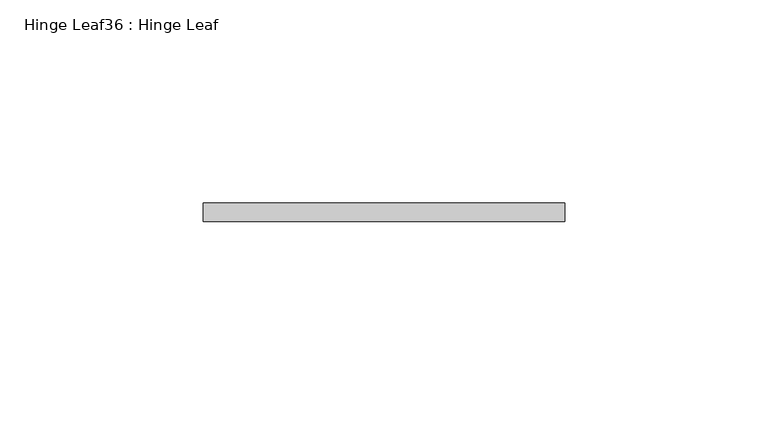
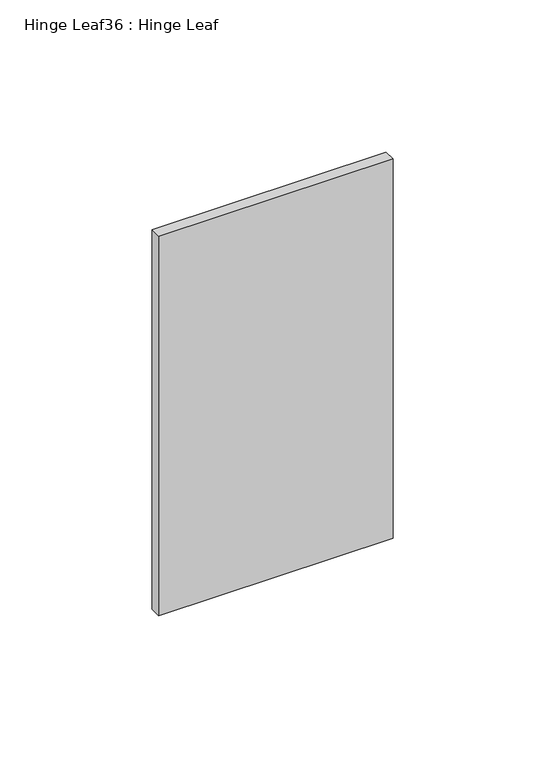
"""IFC4 building model written with IfcOpenShell, lengths in millimetres: proxy geometry, Hinge Leaf36 : Hinge Leaf."""

import ifcopenshell
import ifcopenshell.guid

model = None  # the IFC model being written
_history = None  # IfcOwnerHistory: only IFC2X3 demands one
_inside = {}  # id of a spatial element -> (the spatial element, [elements in it])
_under = {}  # id of a project, library or spatial element -> (it, [spatial elements below it])
_declared = {}  # id of a project -> (the project, [libraries it declares])
_typed = {}  # id of a type object -> (the type object, [elements of that type])
_made_of = {}  # id of a material, layer set ... -> (it, [elements and type objects made of it])


def new_model(schema):
    """Start an empty IFC model of exactly this schema.

    Asked for "IFC4X3", IfcOpenShell would pick the latest addendum, in which some entities
    have other attributes; the version numbers below select the first issue.
    IFC2X3 requires an IfcOwnerHistory on every rooted entity: one is made here for all.
    """
    global model, _history
    if schema == "IFC4X3":
        model = ifcopenshell.file(schema_version=(4, 3, 0, 0))
    else:
        model = ifcopenshell.file(schema=schema)
    _inside.clear()
    _under.clear()
    _declared.clear()
    _typed.clear()
    _made_of.clear()
    _history = None
    if model.schema == "IFC2X3":
        org = make("IfcOrganization", Name="unknown")
        user = make(
            "IfcPersonAndOrganization",
            ThePerson=make("IfcPerson", FamilyName="unknown"),
            TheOrganization=org,
        )
        app = make(
            "IfcApplication",
            ApplicationDeveloper=org,
            Version="unknown",
            ApplicationFullName="unknown",
            ApplicationIdentifier="unknown",
        )
        _history = make(
            "IfcOwnerHistory",
            OwningUser=user,
            OwningApplication=app,
            ChangeAction="ADDED",
            CreationDate=0,
        )
    return model


def make(cls, **values):
    """One entity of the class cls with the attributes given. An attribute that is None is left unset."""
    return model.create_entity(
        cls, **{name: value for name, value in values.items() if value is not None}
    )


def rooted(cls, **values):
    """An entity with a GlobalId (a new one), such as an element, a storey or a relation."""
    return make(cls, GlobalId=ifcopenshell.guid.new(), OwnerHistory=_history, **values)


def si_unit(unit_type, name, prefix=None):
    """IfcSIUnit, for example si_unit("LENGTHUNIT", "METRE", prefix="MILLI")."""
    return make("IfcSIUnit", UnitType=unit_type, Prefix=prefix, Name=name)


def assignment(units):
    """IfcUnitAssignment: the units of a project."""
    return None if units is None else make("IfcUnitAssignment", Units=units)


def point(xyz):
    """IfcCartesianPoint."""
    return None if xyz is None else make("IfcCartesianPoint", Coordinates=xyz)


def direction(xyz):
    """IfcDirection."""
    return None if xyz is None else make("IfcDirection", DirectionRatios=xyz)


def frame(location, z_axis=None, x_axis=None):
    """IfcAxis2Placement3D, a coordinate frame: its origin and axes. An axis left out is left unset."""
    return make(
        "IfcAxis2Placement3D",
        Location=point(location),
        Axis=direction(z_axis),
        RefDirection=direction(x_axis),
    )


def origin():
    """The frame at (0, 0, 0) with its axes left unset."""
    return frame((0.0, 0.0, 0.0))


def place(relative_to, where):
    """IfcLocalPlacement: puts the frame where relative to a parent placement (None: the world)."""
    return make(
        "IfcLocalPlacement", PlacementRelTo=relative_to, RelativePlacement=where
    )


def context(
    kind, dimensions, precision=None, world=None, true_north=None, identifier=None
):
    """IfcGeometricRepresentationContext, for example the 3D "Model" context."""
    return make(
        "IfcGeometricRepresentationContext",
        ContextIdentifier=identifier,
        ContextType=kind,
        CoordinateSpaceDimension=dimensions,
        Precision=precision,
        WorldCoordinateSystem=world,
        TrueNorth=true_north,
    )


def project(units=None, contexts=None):
    """IfcProject with its units and contexts."""
    return rooted(
        "IfcProject",
        Name="project",
        RepresentationContexts=contexts,
        UnitsInContext=assignment(units),
    )


def spatial(cls, under=None, at=None, **own):
    """A site, building, storey or space (cls), placed at a placement, below another one or the project."""
    s = rooted(cls, ObjectPlacement=at, **own)
    if under is not None:
        _under.setdefault(under.id(), (under, []))[1].append(s)
    return s


def polyline(points):
    """IfcPolyline through the points."""
    return make("IfcPolyline", Points=[point(p) for p in points])


def outline(outer, holes=None, kind="AREA"):
    """IfcArbitraryClosedProfileDef: a profile drawn as a closed curve; with holes, ...WithVoids."""
    if holes is None:
        return make("IfcArbitraryClosedProfileDef", ProfileType=kind, OuterCurve=outer)
    return make(
        "IfcArbitraryProfileDefWithVoids",
        ProfileType=kind,
        OuterCurve=outer,
        InnerCurves=holes,
    )


def extrude(swept, where, along, depth):
    """IfcExtrudedAreaSolid: the profile swept, set in the frame where, extruded along a direction by depth."""
    return make(
        "IfcExtrudedAreaSolid",
        SweptArea=swept,
        Position=where,
        ExtrudedDirection=direction(along),
        Depth=depth,
    )


def shape(context_of_items, identifier, shape_type, items):
    """IfcShapeRepresentation: the items that make up one representation, for example the "Body"."""
    return make(
        "IfcShapeRepresentation",
        ContextOfItems=context_of_items,
        RepresentationIdentifier=identifier,
        RepresentationType=shape_type,
        Items=items,
    )


def source(mapping_origin, context_of_items, identifier, shape_type, items):
    """IfcRepresentationMap: a shape defined once, which mapped items show again and again."""
    return make(
        "IfcRepresentationMap",
        MappingOrigin=mapping_origin,
        MappedRepresentation=shape(context_of_items, identifier, shape_type, items),
    )


def transform(
    local_origin,
    x_axis=None,
    y_axis=None,
    z_axis=None,
    scale=None,
    scale2=None,
    scale3=None,
    uniform=True,
):
    """IfcCartesianTransformationOperator3D, or its non-uniform kind. x_axis, y_axis, z_axis: its Axis1, 2, 3."""
    if uniform:
        return make(
            "IfcCartesianTransformationOperator3D",
            Axis1=direction(x_axis),
            Axis2=direction(y_axis),
            LocalOrigin=point(local_origin),
            Scale=scale,
            Axis3=direction(z_axis),
        )
    return make(
        "IfcCartesianTransformationOperator3DnonUniform",
        Axis1=direction(x_axis),
        Axis2=direction(y_axis),
        LocalOrigin=point(local_origin),
        Scale=scale,
        Axis3=direction(z_axis),
        Scale2=scale2,
        Scale3=scale3,
    )


def mapped(mapping_source, mapping_target):
    """IfcMappedItem: shows the shape of a source again, moved by a transform."""
    return make(
        "IfcMappedItem", MappingSource=mapping_source, MappingTarget=mapping_target
    )


def made_of(thing, what):
    """Note that an element or type object is made of a material, layer set ...; save() writes the relation."""
    if what is not None:
        _made_of.setdefault(what.id(), (what, []))[1].append(thing)
    return thing


def element(
    cls,
    number,
    at=None,
    inside=None,
    cuts=None,
    type_object=None,
    material=None,
    context=None,
    identifier="Body",
    shape_type=None,
    held_by="IfcProductDefinitionShape",
    body=None,
    shapes=None,
    **own,
):
    """One element of the class cls, such as IfcWall. Its Tag is "e" and its number.

    at: its placement. inside: the storey or other place that contains it. cuts: it is an
    opening in that element (IfcRelVoidsElement). A single representation is given by context,
    identifier, shape_type and body (its items); several are given by shapes. held_by: the class
    of the entity that holds the representations. save() writes the other relations.
    """
    e = rooted(cls, Tag="e%d" % number, ObjectPlacement=at, **own)
    if body is not None:
        shapes = [shape(context, identifier, shape_type, body)]
    if shapes is not None:
        e.Representation = make(held_by, Representations=shapes)
    if inside is not None:
        _inside.setdefault(inside.id(), (inside, []))[1].append(e)
    if cuts is not None:
        rooted(
            "IfcRelVoidsElement", RelatingBuildingElement=cuts, RelatedOpeningElement=e
        )
    if type_object is not None:
        _typed.setdefault(type_object.id(), (type_object, []))[1].append(e)
    return made_of(e, material)


def aggregate(whole, parts):
    """IfcRelAggregates: a whole, such as a stair, and the parts it consists of."""
    return rooted("IfcRelAggregates", RelatingObject=whole, RelatedObjects=parts)


def save(model, path):
    """Write the relations noted so far, then the file.

    IfcRelAggregates (storeys below a building ...), IfcRelContainedInSpatialStructure (elements
    in a storey), IfcRelDefinesByType, IfcRelAssociatesMaterial and IfcRelDeclares: one each for
    every whole, place, type object, material and project.
    """
    for whole, parts in _under.values():
        aggregate(whole, parts)
    for where, things in _inside.values():
        rooted(
            "IfcRelContainedInSpatialStructure",
            RelatedElements=things,
            RelatingStructure=where,
        )
    for kind, things in _typed.values():
        rooted("IfcRelDefinesByType", RelatedObjects=things, RelatingType=kind)
    for what, things in _made_of.values():
        rooted("IfcRelAssociatesMaterial", RelatedObjects=things, RelatingMaterial=what)
    for by, libraries in _declared.values():
        rooted("IfcRelDeclares", RelatingContext=by, RelatedDefinitions=libraries)
    model.write(path)


def hinge_leaf36_hinge_leaf_05c7f3a5(model_context):
    return source(origin(), model_context, "Body", "SweptSolid", [
        extrude(outline(polyline([(587327.7934739, -533980.5883841), (587327.7934739, -533976.0163841), (587416.6934739, -533976.0163841), (587416.6934739, -533980.5883841), (587327.7934739, -533980.5883841)])), frame((0.0, 0.0, 1123.95), z_axis=(0.0, 0.0, 1.0), x_axis=(1.0, 0.0, 0.0)), (0.0, 0.0, 1.0), 152.4),
    ])


if __name__ == "__main__":
    model = new_model("IFC4")
    model_context = context("Model", 3, world=origin())
    ifc_project = project(units=[si_unit("LENGTHUNIT", "METRE", prefix="MILLI")], contexts=[model_context])
    site = spatial("IfcSite", under=ifc_project)
    building = spatial("IfcBuilding", under=site)
    placement = place(None, origin())
    hinge_leaf36_hinge_leaf_shape = hinge_leaf36_hinge_leaf_05c7f3a5(model_context)
    element("IfcBuildingElementProxy", 1, Name="Hinge Leaf36 : Hinge Leaf", ObjectType="Hinge Leaf36 : Hinge Leaf", at=placement, inside=building, context=model_context, shape_type="MappedRepresentation", body=[
        mapped(hinge_leaf36_hinge_leaf_shape, transform((0.0, 0.0, 0.0), x_axis=(1.0, 0.0, 0.0), y_axis=(0.0, 1.0, 0.0), z_axis=(0.0, 0.0, 1.0))),
    ])
    save(model, "model.ifc")

# Revit data of these elements
# Element 1 (IfcBuildingElementProxy, "Hinge Leaf36 : Hinge Leaf")
#   Materials on its faces: "6\"X6\" WELD-ON STL BUTT HINGE"
# Materials
#   "6\"X6\" WELD-ON STL BUTT HINGE": class "Metal", colour RGB 189 187 185, transparency 0, Description = "Carbon steel", Cost = 0
